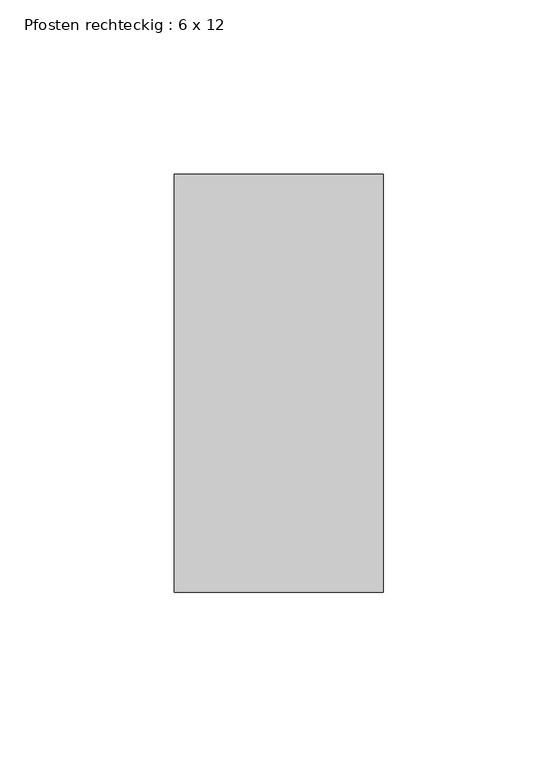
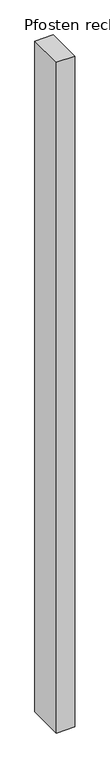
"""IFC4 building model written with IfcOpenShell, lengths in millimetres: member geometry, Pfosten rechteckig : 6 x 12."""

from ifc_helpers import new_model, si_unit, frame, origin, place, context, project, spatial, polyline, outline, extrude, source, transform, mapped, element, save


def pfosten_rechteckig_6_x_12_74b065d3(model_context):
    return source(origin(), model_context, "Body", "SweptSolid", [
        extrude(outline(polyline([(0.0, 60.0), (0.0, -60.0), (-60.0, -60.0), (-60.0, 60.0), (0.0, 60.0)])), frame((0.0, 0.0, -2290.8558388), z_axis=(0.0, 0.0, 1.0), x_axis=(1.0, 0.0, 0.0)), (0.0, 0.0, 1.0), 2290.8558388),
    ])


if __name__ == "__main__":
    model = new_model("IFC4")
    model_context = context("Model", 3, world=origin())
    ifc_project = project(units=[si_unit("LENGTHUNIT", "METRE", prefix="MILLI")], contexts=[model_context])
    site = spatial("IfcSite", under=ifc_project)
    building = spatial("IfcBuilding", under=site)
    placement = place(None, origin())
    pfosten_rechteckig_6_x_12_shape = pfosten_rechteckig_6_x_12_74b065d3(model_context)
    element("IfcMember", 1, ObjectType="Pfosten rechteckig : 6 x 12", at=placement, inside=building, context=model_context, shape_type="MappedRepresentation", body=[
        mapped(pfosten_rechteckig_6_x_12_shape, transform((0.0, 0.0, 0.0), x_axis=(1.0, 0.0, 0.0), y_axis=(0.0, 1.0, 0.0), z_axis=(0.0, 0.0, 1.0))),
    ])
    save(model, "model.ifc")

# Revit data of these elements
# Type "Pfosten rechteckig : 6 x 12"
#   built-in parameter 1007304 = 0.393701 (stored number, unit not read)
#   built-in parameter 1007301 = 0.0984252 (stored number, unit not read)
#   built-in parameter 1007300 = 0.0984252 (stored number, unit not read)
# Element 1 (IfcMember, "Pfosten rechteckig : 6 x 12")
#   Materials on its faces: "Metall - verzinkt"
# Materials
#   "Metall - verzinkt": class "Allgemeines", colour RGB 200 200 200, transparency 0, Cost = 0
